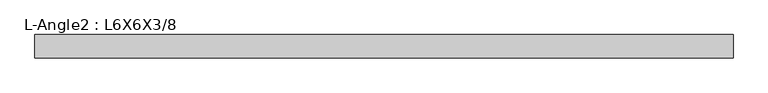
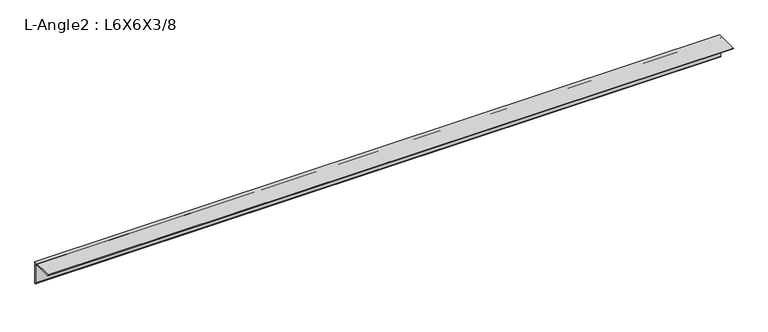
"""IFC4 building model written with IfcOpenShell, lengths in millimetres: member geometry, L-Angle2 : L6X6X3/8."""

from ifc_helpers import new_model, si_unit, point, frame, frame_2d, origin, place, context, project, spatial, polyline, circle_curve, trimmed, segment, composite_curve, outline, extrude, source, transform, mapped, element, save


def l_angle2_l6x6x3_8_34c47d6c(model_context):
    return source(origin(), model_context, "Body", "SweptSolid", [
        extrude(outline(composite_curve([segment(polyline([(41.148, 41.148), (41.148, -111.252)]), True, "CONTINUOUS"), segment(trimmed(circle_curve(frame_2d((41.148, -101.727)), 9.525), [point((41.148, -111.252))], [point((31.623, -101.727))], False, "CARTESIAN"), True, "CONTINUOUS"), segment(polyline([(31.623, -101.727), (31.623, 22.098)]), True, "CONTINUOUS"), segment(trimmed(circle_curve(frame_2d((22.098, 22.098)), 9.525), [point((31.623, 22.098))], [point((22.098, 31.623))], True, "CARTESIAN"), True, "CONTINUOUS"), segment(polyline([(22.098, 31.623), (-101.727, 31.623)]), True, "CONTINUOUS"), segment(trimmed(circle_curve(frame_2d((-101.727, 41.148)), 9.525), [point((-101.727, 31.623))], [point((-111.252, 41.148))], False, "CARTESIAN"), True, "CONTINUOUS"), segment(polyline([(-111.252, 41.148), (41.148, 41.148)]), True, "CONTINUOUS")], self_intersect=False)), frame((-2289.5946037, 0.0, 0.0), z_axis=(1.0, 0.0, 0.0), x_axis=(0.0, 1.0, 0.0)), (0.0, 0.0, 1.0), 4540.0613934),
    ])


if __name__ == "__main__":
    model = new_model("IFC4")
    model_context = context("Model", 3, world=origin())
    ifc_project = project(units=[si_unit("LENGTHUNIT", "METRE", prefix="MILLI")], contexts=[model_context])
    site = spatial("IfcSite", under=ifc_project)
    building = spatial("IfcBuilding", under=site)
    placement = place(None, origin())
    l_angle2_l6x6x3_8_shape = l_angle2_l6x6x3_8_34c47d6c(model_context)
    element("IfcMember", 1, ObjectType="L-Angle2 : L6X6X3/8", at=placement, inside=building, context=model_context, shape_type="MappedRepresentation", body=[
        mapped(l_angle2_l6x6x3_8_shape, transform((0.0, 0.0, 0.0), x_axis=(1.0, 0.0, 0.0), y_axis=(0.0, 1.0, 0.0), z_axis=(0.0, 0.0, 1.0))),
    ])
    save(model, "model.ifc")

# Revit data of these elements
# Type "L-Angle2 : L6X6X3/8"
#   Assembly Code = "B10"
#   k = 0' - 0 7/8"
#   W = 14.9
#   Length [instance default] = 5' - 0"
#   b = 0' - 6"
#   d = 0' - 6"
#   t = 0' - 0 3/8"
#   x = 0' - 1.62"
#   y = 0' - 1.62"
#   A = 0.0304167 SF
#   Structural Material [instance default] = Steel ASTM A36
# Element 1 (IfcMember, "L-Angle2 : L6X6X3/8")
#   Materials on its faces: "Steel ASTM A36"
# Materials
#   "Steel ASTM A36": class "Metal", colour RGB 199 199 199, transparency 0, Description = "Structural steel, ASTM A36 Grade B, mill finish", Cost = 0
